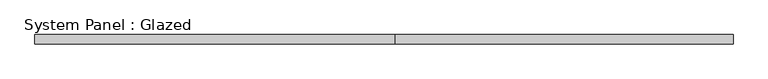
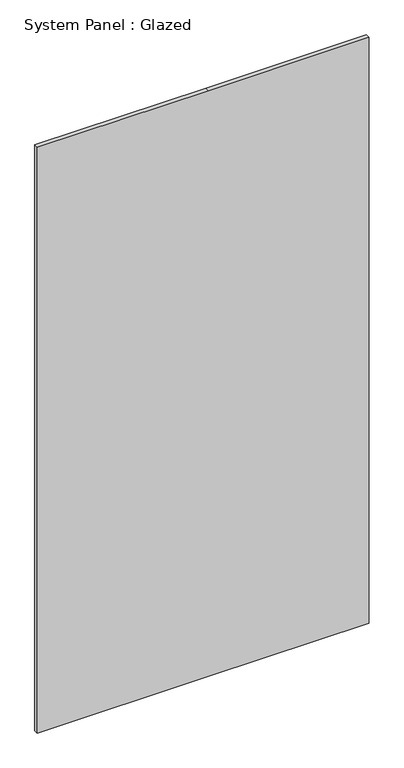
"""IFC4 building model written with IfcOpenShell, lengths in millimetres: plate geometry, System Panel : Glazed."""

import ifcopenshell
import ifcopenshell.guid

model = None  # the IFC model being written
_history = None  # IfcOwnerHistory: only IFC2X3 demands one
_inside = {}  # id of a spatial element -> (the spatial element, [elements in it])
_under = {}  # id of a project, library or spatial element -> (it, [spatial elements below it])
_declared = {}  # id of a project -> (the project, [libraries it declares])
_typed = {}  # id of a type object -> (the type object, [elements of that type])
_made_of = {}  # id of a material, layer set ... -> (it, [elements and type objects made of it])


def new_model(schema):
    """Start an empty IFC model of exactly this schema.

    Asked for "IFC4X3", IfcOpenShell would pick the latest addendum, in which some entities
    have other attributes; the version numbers below select the first issue.
    IFC2X3 requires an IfcOwnerHistory on every rooted entity: one is made here for all.
    """
    global model, _history
    if schema == "IFC4X3":
        model = ifcopenshell.file(schema_version=(4, 3, 0, 0))
    else:
        model = ifcopenshell.file(schema=schema)
    _inside.clear()
    _under.clear()
    _declared.clear()
    _typed.clear()
    _made_of.clear()
    _history = None
    if model.schema == "IFC2X3":
        org = make("IfcOrganization", Name="unknown")
        user = make(
            "IfcPersonAndOrganization",
            ThePerson=make("IfcPerson", FamilyName="unknown"),
            TheOrganization=org,
        )
        app = make(
            "IfcApplication",
            ApplicationDeveloper=org,
            Version="unknown",
            ApplicationFullName="unknown",
            ApplicationIdentifier="unknown",
        )
        _history = make(
            "IfcOwnerHistory",
            OwningUser=user,
            OwningApplication=app,
            ChangeAction="ADDED",
            CreationDate=0,
        )
    return model


def make(cls, **values):
    """One entity of the class cls with the attributes given. An attribute that is None is left unset."""
    return model.create_entity(
        cls, **{name: value for name, value in values.items() if value is not None}
    )


def rooted(cls, **values):
    """An entity with a GlobalId (a new one), such as an element, a storey or a relation."""
    return make(cls, GlobalId=ifcopenshell.guid.new(), OwnerHistory=_history, **values)


def si_unit(unit_type, name, prefix=None):
    """IfcSIUnit, for example si_unit("LENGTHUNIT", "METRE", prefix="MILLI")."""
    return make("IfcSIUnit", UnitType=unit_type, Prefix=prefix, Name=name)


def assignment(units):
    """IfcUnitAssignment: the units of a project."""
    return None if units is None else make("IfcUnitAssignment", Units=units)


def point(xyz):
    """IfcCartesianPoint."""
    return None if xyz is None else make("IfcCartesianPoint", Coordinates=xyz)


def direction(xyz):
    """IfcDirection."""
    return None if xyz is None else make("IfcDirection", DirectionRatios=xyz)


def frame(location, z_axis=None, x_axis=None):
    """IfcAxis2Placement3D, a coordinate frame: its origin and axes. An axis left out is left unset."""
    return make(
        "IfcAxis2Placement3D",
        Location=point(location),
        Axis=direction(z_axis),
        RefDirection=direction(x_axis),
    )


def origin():
    """The frame at (0, 0, 0) with its axes left unset."""
    return frame((0.0, 0.0, 0.0))


def place(relative_to, where):
    """IfcLocalPlacement: puts the frame where relative to a parent placement (None: the world)."""
    return make(
        "IfcLocalPlacement", PlacementRelTo=relative_to, RelativePlacement=where
    )


def context(
    kind, dimensions, precision=None, world=None, true_north=None, identifier=None
):
    """IfcGeometricRepresentationContext, for example the 3D "Model" context."""
    return make(
        "IfcGeometricRepresentationContext",
        ContextIdentifier=identifier,
        ContextType=kind,
        CoordinateSpaceDimension=dimensions,
        Precision=precision,
        WorldCoordinateSystem=world,
        TrueNorth=true_north,
    )


def project(units=None, contexts=None):
    """IfcProject with its units and contexts."""
    return rooted(
        "IfcProject",
        Name="project",
        RepresentationContexts=contexts,
        UnitsInContext=assignment(units),
    )


def spatial(cls, under=None, at=None, **own):
    """A site, building, storey or space (cls), placed at a placement, below another one or the project."""
    s = rooted(cls, ObjectPlacement=at, **own)
    if under is not None:
        _under.setdefault(under.id(), (under, []))[1].append(s)
    return s


def polyline(points):
    """IfcPolyline through the points."""
    return make("IfcPolyline", Points=[point(p) for p in points])


def outline(outer, holes=None, kind="AREA"):
    """IfcArbitraryClosedProfileDef: a profile drawn as a closed curve; with holes, ...WithVoids."""
    if holes is None:
        return make("IfcArbitraryClosedProfileDef", ProfileType=kind, OuterCurve=outer)
    return make(
        "IfcArbitraryProfileDefWithVoids",
        ProfileType=kind,
        OuterCurve=outer,
        InnerCurves=holes,
    )


def extrude(swept, where, along, depth):
    """IfcExtrudedAreaSolid: the profile swept, set in the frame where, extruded along a direction by depth."""
    return make(
        "IfcExtrudedAreaSolid",
        SweptArea=swept,
        Position=where,
        ExtrudedDirection=direction(along),
        Depth=depth,
    )


def shape(context_of_items, identifier, shape_type, items):
    """IfcShapeRepresentation: the items that make up one representation, for example the "Body"."""
    return make(
        "IfcShapeRepresentation",
        ContextOfItems=context_of_items,
        RepresentationIdentifier=identifier,
        RepresentationType=shape_type,
        Items=items,
    )


def source(mapping_origin, context_of_items, identifier, shape_type, items):
    """IfcRepresentationMap: a shape defined once, which mapped items show again and again."""
    return make(
        "IfcRepresentationMap",
        MappingOrigin=mapping_origin,
        MappedRepresentation=shape(context_of_items, identifier, shape_type, items),
    )


def transform(
    local_origin,
    x_axis=None,
    y_axis=None,
    z_axis=None,
    scale=None,
    scale2=None,
    scale3=None,
    uniform=True,
):
    """IfcCartesianTransformationOperator3D, or its non-uniform kind. x_axis, y_axis, z_axis: its Axis1, 2, 3."""
    if uniform:
        return make(
            "IfcCartesianTransformationOperator3D",
            Axis1=direction(x_axis),
            Axis2=direction(y_axis),
            LocalOrigin=point(local_origin),
            Scale=scale,
            Axis3=direction(z_axis),
        )
    return make(
        "IfcCartesianTransformationOperator3DnonUniform",
        Axis1=direction(x_axis),
        Axis2=direction(y_axis),
        LocalOrigin=point(local_origin),
        Scale=scale,
        Axis3=direction(z_axis),
        Scale2=scale2,
        Scale3=scale3,
    )


def mapped(mapping_source, mapping_target):
    """IfcMappedItem: shows the shape of a source again, moved by a transform."""
    return make(
        "IfcMappedItem", MappingSource=mapping_source, MappingTarget=mapping_target
    )


def made_of(thing, what):
    """Note that an element or type object is made of a material, layer set ...; save() writes the relation."""
    if what is not None:
        _made_of.setdefault(what.id(), (what, []))[1].append(thing)
    return thing


def element(
    cls,
    number,
    at=None,
    inside=None,
    cuts=None,
    type_object=None,
    material=None,
    context=None,
    identifier="Body",
    shape_type=None,
    held_by="IfcProductDefinitionShape",
    body=None,
    shapes=None,
    **own,
):
    """One element of the class cls, such as IfcWall. Its Tag is "e" and its number.

    at: its placement. inside: the storey or other place that contains it. cuts: it is an
    opening in that element (IfcRelVoidsElement). A single representation is given by context,
    identifier, shape_type and body (its items); several are given by shapes. held_by: the class
    of the entity that holds the representations. save() writes the other relations.
    """
    e = rooted(cls, Tag="e%d" % number, ObjectPlacement=at, **own)
    if body is not None:
        shapes = [shape(context, identifier, shape_type, body)]
    if shapes is not None:
        e.Representation = make(held_by, Representations=shapes)
    if inside is not None:
        _inside.setdefault(inside.id(), (inside, []))[1].append(e)
    if cuts is not None:
        rooted(
            "IfcRelVoidsElement", RelatingBuildingElement=cuts, RelatedOpeningElement=e
        )
    if type_object is not None:
        _typed.setdefault(type_object.id(), (type_object, []))[1].append(e)
    return made_of(e, material)


def aggregate(whole, parts):
    """IfcRelAggregates: a whole, such as a stair, and the parts it consists of."""
    return rooted("IfcRelAggregates", RelatingObject=whole, RelatedObjects=parts)


def save(model, path):
    """Write the relations noted so far, then the file.

    IfcRelAggregates (storeys below a building ...), IfcRelContainedInSpatialStructure (elements
    in a storey), IfcRelDefinesByType, IfcRelAssociatesMaterial and IfcRelDeclares: one each for
    every whole, place, type object, material and project.
    """
    for whole, parts in _under.values():
        aggregate(whole, parts)
    for where, things in _inside.values():
        rooted(
            "IfcRelContainedInSpatialStructure",
            RelatedElements=things,
            RelatingStructure=where,
        )
    for kind, things in _typed.values():
        rooted("IfcRelDefinesByType", RelatedObjects=things, RelatingType=kind)
    for what, things in _made_of.values():
        rooted("IfcRelAssociatesMaterial", RelatedObjects=things, RelatingMaterial=what)
    for by, libraries in _declared.values():
        rooted("IfcRelDeclares", RelatingContext=by, RelatedDefinitions=libraries)
    model.write(path)


def system_panel_glazed_cbecbb20(model_context):
    return source(origin(), model_context, "Body", "SweptSolid", [
        extrude(outline(polyline([(0.0, -971.55), (0.0, 31.75), (0.0, 971.55), (3625.85, 971.55), (3625.85, 31.75), (3625.85, -971.55), (0.0, -971.55)])), frame((0.0, -44.45, 0.0), z_axis=(0.0, 1.0, 0.0), x_axis=(0.0, 0.0, 1.0)), (0.0, 0.0, 1.0), 25.4),
    ])


if __name__ == "__main__":
    model = new_model("IFC4")
    model_context = context("Model", 3, world=origin())
    ifc_project = project(units=[si_unit("LENGTHUNIT", "METRE", prefix="MILLI")], contexts=[model_context])
    site = spatial("IfcSite", under=ifc_project)
    building = spatial("IfcBuilding", under=site)
    placement = place(None, origin())
    system_panel_glazed_shape = system_panel_glazed_cbecbb20(model_context)
    element("IfcPlate", 1, ObjectType="System Panel : Glazed", at=placement, inside=building, context=model_context, shape_type="MappedRepresentation", body=[
        mapped(system_panel_glazed_shape, transform((0.0, 0.0, 0.0), x_axis=(1.0, 0.0, 0.0), y_axis=(0.0, 1.0, 0.0), z_axis=(0.0, 0.0, 1.0))),
    ])
    save(model, "model.ifc")

# Revit data of these elements
# Element 1 (IfcPlate, "System Panel : Glazed")
#   Materials on its faces: "Glass"
# Materials
#   "Glass": class "Unassigned", colour RGB 0 0 255, transparency 0.75
